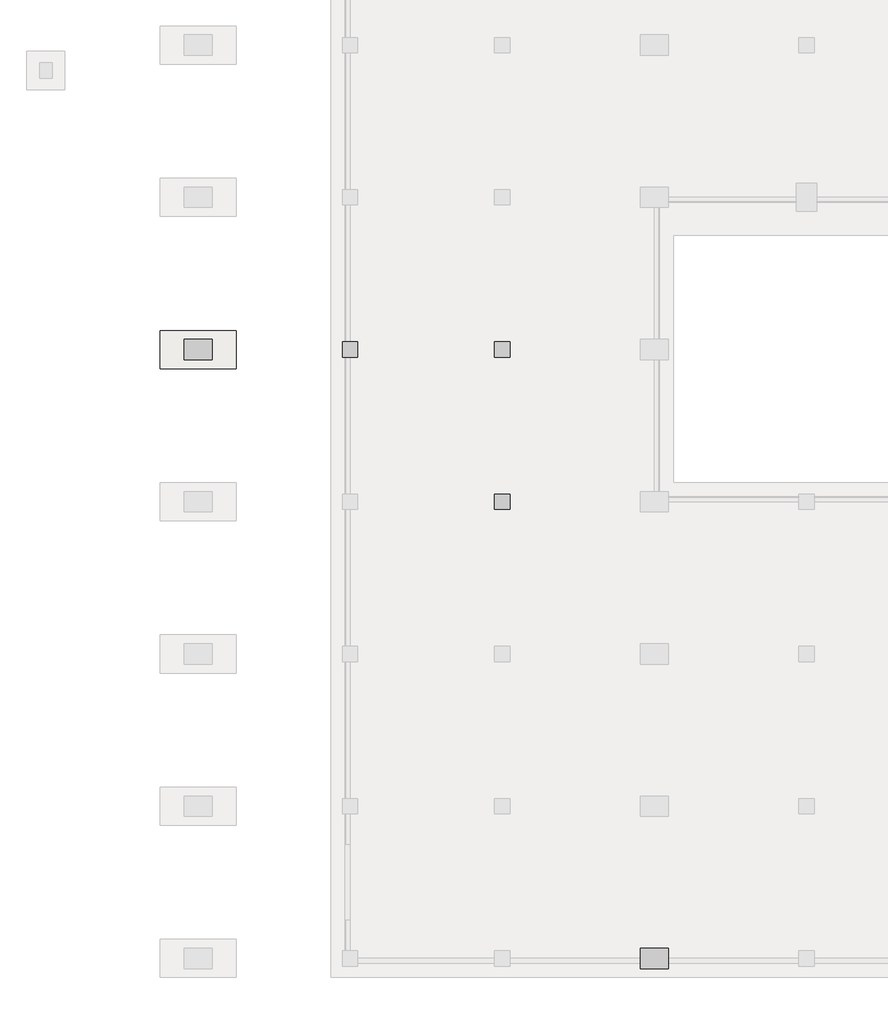
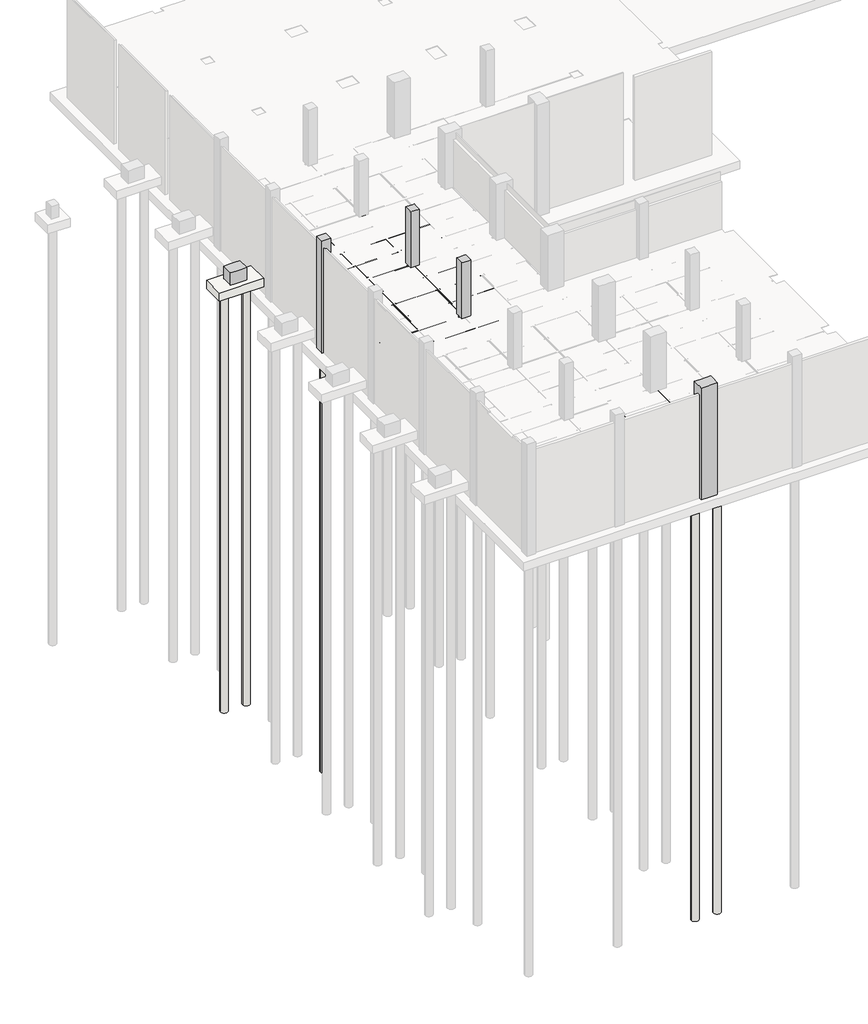
# Not in any storey, part 3 of 16: 28 beams, 6 slabs, 5 columns.
"""IFC4 building model written with IfcOpenShell, lengths in millimetres."""

from ifc_helpers import new_model, si_unit, point, frame, frame_2d, origin, place, context, project, spatial, polyline, circle_curve, trimmed, segment, composite_curve, outline, extrude, faceted_brep, element, save

model = new_model("IFC4")

# Units and contexts
model_context = context("Model", 3, world=origin())
ifc_project = project(units=[si_unit("LENGTHUNIT", "METRE", prefix="MILLI")], contexts=[model_context])

# Site, building
site = spatial("IfcSite", under=ifc_project)
building = spatial("IfcBuilding", under=site)

# Beams
placement = place(None, origin())
element("IfcBeam", 1, ObjectType="Steel Framing_C_KS : H_SB_AR_S02_C-150x75x6.5x10_J1", at=placement, inside=building, context=model_context, shape_type="SweptSolid", body=[
    extrude(outline(composite_curve([segment(polyline([(-43477.2, -3800.0381366), (-43477.2, -3950.0381366), (-43552.2, -3950.0381366)]), True, "CONTINUOUS"), segment(trimmed(circle_curve(frame_2d((-43542.2, -3950.0381366)), 10.0), [point((-43552.2, -3950.0381366))], [point((-43542.2, -3940.0381366))], False, "CARTESIAN"), True, "CONTINUOUS"), segment(polyline([(-43542.2, -3940.0381366), (-43483.7, -3930.7726469), (-43483.7, -3819.3036264), (-43542.2, -3810.0381366)]), True, "CONTINUOUS"), segment(trimmed(circle_curve(frame_2d((-43542.2, -3800.0381366)), 10.0), [point((-43542.2, -3810.0381366))], [point((-43552.2, -3800.0381366))], False, "CARTESIAN"), True, "CONTINUOUS"), segment(polyline([(-43552.2, -3800.0381366), (-43477.2, -3800.0381366)]), True, "CONTINUOUS")], self_intersect=False)), frame((27112.7, 0.0, 0.0), z_axis=(1.0, 0.0, 0.0), x_axis=(0.0, 1.0, 0.0)), (0.0, 0.0, 1.0), 2774.6),
])
element("IfcBeam", 2, ObjectType="Steel Framing_C_KS : H_SB_AR_S02_C-150x75x6.5x10_J1", at=placement, inside=building, context=model_context, shape_type="SweptSolid", body=[
    extrude(outline(composite_curve([segment(polyline([(-43477.2, -3800.0381366), (-43477.2, -3950.0381366), (-43552.2, -3950.0381366)]), True, "CONTINUOUS"), segment(trimmed(circle_curve(frame_2d((-43542.2, -3950.0381366)), 10.0), [point((-43552.2, -3950.0381366))], [point((-43542.2, -3940.0381366))], False, "CARTESIAN"), True, "CONTINUOUS"), segment(polyline([(-43542.2, -3940.0381366), (-43483.7, -3930.7726469), (-43483.7, -3819.3036264), (-43542.2, -3810.0381366)]), True, "CONTINUOUS"), segment(trimmed(circle_curve(frame_2d((-43542.2, -3800.0381366)), 10.0), [point((-43542.2, -3810.0381366))], [point((-43552.2, -3800.0381366))], False, "CARTESIAN"), True, "CONTINUOUS"), segment(polyline([(-43552.2, -3800.0381366), (-43477.2, -3800.0381366)]), True, "CONTINUOUS")], self_intersect=False)), frame((30112.7, 0.0, 0.0), z_axis=(1.0, 0.0, 0.0), x_axis=(0.0, 1.0, 0.0)), (0.0, 0.0, 1.0), 2774.6),
])
element("IfcBeam", 3, ObjectType="Steel Framing_H_KS : H_SB_AR_S02_H-400x200x8x13_BSG2", at=placement, inside=building, context=model_context, shape_type="SweptSolid", body=[
    extrude(outline(composite_curve([segment(polyline([(-4187.0381366, 35900.0), (-4200.0381366, 35900.0), (-4200.0381366, 36100.0), (-4187.0381366, 36100.0), (-4187.0381366, 36020.0)]), True, "CONTINUOUS"), segment(trimmed(circle_curve(frame_2d((-4171.0381366, 36020.0)), 16.0), [point((-4187.0381366, 36020.0))], [point((-4171.0381366, 36004.0))], True, "CARTESIAN"), True, "CONTINUOUS"), segment(polyline([(-4171.0381366, 36004.0), (-3829.0381366, 36004.0)]), True, "CONTINUOUS"), segment(trimmed(circle_curve(frame_2d((-3829.0381366, 36020.0)), 16.0), [point((-3829.0381366, 36004.0))], [point((-3813.0381366, 36020.0))], True, "CARTESIAN"), True, "CONTINUOUS"), segment(polyline([(-3813.0381366, 36020.0), (-3813.0381366, 36100.0), (-3800.0381366, 36100.0), (-3800.0381366, 35900.0), (-3813.0381366, 35900.0), (-3813.0381366, 35980.0)]), True, "CONTINUOUS"), segment(trimmed(circle_curve(frame_2d((-3829.0381366, 35980.0)), 16.0), [point((-3813.0381366, 35980.0))], [point((-3829.0381366, 35996.0))], True, "CARTESIAN"), True, "CONTINUOUS"), segment(polyline([(-3829.0381366, 35996.0), (-4171.0381366, 35996.0)]), True, "CONTINUOUS"), segment(trimmed(circle_curve(frame_2d((-4171.0381366, 35980.0)), 16.0), [point((-4171.0381366, 35996.0))], [point((-4187.0381366, 35980.0))], True, "CARTESIAN"), True, "CONTINUOUS"), segment(polyline([(-4187.0381366, 35980.0), (-4187.0381366, 35900.0)]), True, "CONTINUOUS")], self_intersect=False)), frame((0.0, -59587.3, 0.0), z_axis=(0.0, 1.0, 0.0), x_axis=(0.0, 0.0, 1.0)), (0.0, 0.0, 1.0), 5174.6),
])
element("IfcBeam", 4, ObjectType="Steel Framing_H_KS : H_SB_AR_S02_H-400x200x8x13_BSB1", at=placement, inside=building, context=model_context, shape_type="SweptSolid", body=[
    extrude(outline(composite_curve([segment(polyline([(-4187.0381366, 32900.0), (-4200.0381366, 32900.0), (-4200.0381366, 33100.0), (-4187.0381366, 33100.0), (-4187.0381366, 33020.0)]), True, "CONTINUOUS"), segment(trimmed(circle_curve(frame_2d((-4171.0381366, 33020.0)), 16.0), [point((-4187.0381366, 33020.0))], [point((-4171.0381366, 33004.0))], True, "CARTESIAN"), True, "CONTINUOUS"), segment(polyline([(-4171.0381366, 33004.0), (-3829.0381366, 33004.0)]), True, "CONTINUOUS"), segment(trimmed(circle_curve(frame_2d((-3829.0381366, 33020.0)), 16.0), [point((-3829.0381366, 33004.0))], [point((-3813.0381366, 33020.0))], True, "CARTESIAN"), True, "CONTINUOUS"), segment(polyline([(-3813.0381366, 33020.0), (-3813.0381366, 33100.0), (-3800.0381366, 33100.0), (-3800.0381366, 32900.0), (-3813.0381366, 32900.0), (-3813.0381366, 32980.0)]), True, "CONTINUOUS"), segment(trimmed(circle_curve(frame_2d((-3829.0381366, 32980.0)), 16.0), [point((-3813.0381366, 32980.0))], [point((-3829.0381366, 32996.0))], True, "CARTESIAN"), True, "CONTINUOUS"), segment(polyline([(-3829.0381366, 32996.0), (-4171.0381366, 32996.0)]), True, "CONTINUOUS"), segment(trimmed(circle_curve(frame_2d((-4171.0381366, 32980.0)), 16.0), [point((-4171.0381366, 32996.0))], [point((-4187.0381366, 32980.0))], True, "CARTESIAN"), True, "CONTINUOUS"), segment(polyline([(-4187.0381366, 32980.0), (-4187.0381366, 32900.0)]), True, "CONTINUOUS")], self_intersect=False)), frame((0.0, -60000.0, 0.0), z_axis=(0.0, 1.0, 0.0), x_axis=(0.0, 0.0, 1.0)), (0.0, 0.0, 1.0), 5887.3),
])
element("IfcBeam", 5, ObjectType="Steel Framing_C_KS : H_SB_AR_S02_C-150x75x6.5x10_J1", at=placement, inside=building, context=model_context, shape_type="SweptSolid", body=[
    extrude(outline(composite_curve([segment(polyline([(-56977.2, -3800.0381366), (-56977.2, -3950.0381366), (-57052.2, -3950.0381366)]), True, "CONTINUOUS"), segment(trimmed(circle_curve(frame_2d((-57042.2, -3950.0381366)), 10.0), [point((-57052.2, -3950.0381366))], [point((-57042.2, -3940.0381366))], False, "CARTESIAN"), True, "CONTINUOUS"), segment(polyline([(-57042.2, -3940.0381366), (-56983.7, -3930.7726469), (-56983.7, -3819.3036264), (-57042.2, -3810.0381366)]), True, "CONTINUOUS"), segment(trimmed(circle_curve(frame_2d((-57042.2, -3800.0381366)), 10.0), [point((-57042.2, -3810.0381366))], [point((-57052.2, -3800.0381366))], False, "CARTESIAN"), True, "CONTINUOUS"), segment(polyline([(-57052.2, -3800.0381366), (-56977.2, -3800.0381366)]), True, "CONTINUOUS")], self_intersect=False)), frame((33112.7, 0.0, 0.0), z_axis=(1.0, 0.0, 0.0), x_axis=(0.0, 1.0, 0.0)), (0.0, 0.0, 1.0), 2774.6),
])
element("IfcBeam", 6, ObjectType="Steel Framing_C_KS : H_SB_AR_S02_C-150x75x6.5x10_J1", at=placement, inside=building, context=model_context, shape_type="SweptSolid", body=[
    extrude(outline(composite_curve([segment(polyline([(-58477.2, -3800.0381366), (-58477.2, -3950.0381366), (-58552.2, -3950.0381366)]), True, "CONTINUOUS"), segment(trimmed(circle_curve(frame_2d((-58542.2, -3950.0381366)), 10.0), [point((-58552.2, -3950.0381366))], [point((-58542.2, -3940.0381366))], False, "CARTESIAN"), True, "CONTINUOUS"), segment(polyline([(-58542.2, -3940.0381366), (-58483.7, -3930.7726469), (-58483.7, -3819.3036264), (-58542.2, -3810.0381366)]), True, "CONTINUOUS"), segment(trimmed(circle_curve(frame_2d((-58542.2, -3800.0381366)), 10.0), [point((-58542.2, -3810.0381366))], [point((-58552.2, -3800.0381366))], False, "CARTESIAN"), True, "CONTINUOUS"), segment(polyline([(-58552.2, -3800.0381366), (-58477.2, -3800.0381366)]), True, "CONTINUOUS")], self_intersect=False)), frame((33112.7, 0.0, 0.0), z_axis=(1.0, 0.0, 0.0), x_axis=(0.0, 1.0, 0.0)), (0.0, 0.0, 1.0), 2774.6),
])
element("IfcBeam", 7, ObjectType="Steel Framing_C_KS : H_SB_AR_S02_C-150x75x6.5x10_J1", at=placement, inside=building, context=model_context, shape_type="SweptSolid", body=[
    extrude(outline(composite_curve([segment(polyline([(-56977.2, -3800.0381366), (-56977.2, -3950.0381366), (-57052.2, -3950.0381366)]), True, "CONTINUOUS"), segment(trimmed(circle_curve(frame_2d((-57042.2, -3950.0381366)), 10.0), [point((-57052.2, -3950.0381366))], [point((-57042.2, -3940.0381366))], False, "CARTESIAN"), True, "CONTINUOUS"), segment(polyline([(-57042.2, -3940.0381366), (-56983.7, -3930.7726469), (-56983.7, -3819.3036264), (-57042.2, -3810.0381366)]), True, "CONTINUOUS"), segment(trimmed(circle_curve(frame_2d((-57042.2, -3800.0381366)), 10.0), [point((-57042.2, -3810.0381366))], [point((-57052.2, -3800.0381366))], False, "CARTESIAN"), True, "CONTINUOUS"), segment(polyline([(-57052.2, -3800.0381366), (-56977.2, -3800.0381366)]), True, "CONTINUOUS")], self_intersect=False)), frame((36112.7, 0.0, 0.0), z_axis=(1.0, 0.0, 0.0), x_axis=(0.0, 1.0, 0.0)), (0.0, 0.0, 1.0), 2774.6),
])
element("IfcBeam", 8, ObjectType="Steel Framing_C_KS : H_SB_AR_S02_C-150x75x6.5x10_J1", at=placement, inside=building, context=model_context, shape_type="SweptSolid", body=[
    extrude(outline(composite_curve([segment(polyline([(-58477.2, -3800.0381366), (-58477.2, -3950.0381366), (-58552.2, -3950.0381366)]), True, "CONTINUOUS"), segment(trimmed(circle_curve(frame_2d((-58542.2, -3950.0381366)), 10.0), [point((-58552.2, -3950.0381366))], [point((-58542.2, -3940.0381366))], False, "CARTESIAN"), True, "CONTINUOUS"), segment(polyline([(-58542.2, -3940.0381366), (-58483.7, -3930.7726469), (-58483.7, -3819.3036264), (-58542.2, -3810.0381366)]), True, "CONTINUOUS"), segment(trimmed(circle_curve(frame_2d((-58542.2, -3800.0381366)), 10.0), [point((-58542.2, -3810.0381366))], [point((-58552.2, -3800.0381366))], False, "CARTESIAN"), True, "CONTINUOUS"), segment(polyline([(-58552.2, -3800.0381366), (-58477.2, -3800.0381366)]), True, "CONTINUOUS")], self_intersect=False)), frame((36112.7, 0.0, 0.0), z_axis=(1.0, 0.0, 0.0), x_axis=(0.0, 1.0, 0.0)), (0.0, 0.0, 1.0), 2774.6),
])
element("IfcBeam", 9, ObjectType="Steel Framing_H_KS : H_SB_AR_S02_H-400x200x8x13_BSG1", at=placement, inside=building, context=model_context, shape_type="SweptSolid", body=[
    extrude(outline(composite_curve([segment(polyline([(-35900.0, -4187.0381366), (-35900.0, -4200.0381366), (-36100.0, -4200.0381366), (-36100.0, -4187.0381366), (-36020.0, -4187.0381366)]), True, "CONTINUOUS"), segment(trimmed(circle_curve(frame_2d((-36020.0, -4171.0381366)), 16.0), [point((-36020.0, -4187.0381366))], [point((-36004.0, -4171.0381366))], True, "CARTESIAN"), True, "CONTINUOUS"), segment(polyline([(-36004.0, -4171.0381366), (-36004.0, -3829.0381366)]), True, "CONTINUOUS"), segment(trimmed(circle_curve(frame_2d((-36020.0, -3829.0381366)), 16.0), [point((-36004.0, -3829.0381366))], [point((-36020.0, -3813.0381366))], True, "CARTESIAN"), True, "CONTINUOUS"), segment(polyline([(-36020.0, -3813.0381366), (-36100.0, -3813.0381366), (-36100.0, -3800.0381366), (-35900.0, -3800.0381366), (-35900.0, -3813.0381366), (-35980.0, -3813.0381366)]), True, "CONTINUOUS"), segment(trimmed(circle_curve(frame_2d((-35980.0, -3829.0381366)), 16.0), [point((-35980.0, -3813.0381366))], [point((-35996.0, -3829.0381366))], True, "CARTESIAN"), True, "CONTINUOUS"), segment(polyline([(-35996.0, -3829.0381366), (-35996.0, -4171.0381366)]), True, "CONTINUOUS"), segment(trimmed(circle_curve(frame_2d((-35980.0, -4171.0381366)), 16.0), [point((-35996.0, -4171.0381366))], [point((-35980.0, -4187.0381366))], True, "CARTESIAN"), True, "CONTINUOUS"), segment(polyline([(-35980.0, -4187.0381366), (-35900.0, -4187.0381366)]), True, "CONTINUOUS")], self_intersect=False)), frame((24312.7, 0.0, 0.0), z_axis=(1.0, 0.0, 0.0), x_axis=(0.0, 1.0, 0.0)), (0.0, 0.0, 1.0), 5374.6),
])
element("IfcBeam", 10, ObjectType="Steel Framing_H_KS : H_SB_AR_S02_H-400x200x8x13_BSG2", at=placement, inside=building, context=model_context, shape_type="SweptSolid", body=[
    extrude(outline(composite_curve([segment(polyline([(-4187.0381366, 29900.0), (-4200.0381366, 29900.0), (-4200.0381366, 30100.0), (-4187.0381366, 30100.0), (-4187.0381366, 30020.0)]), True, "CONTINUOUS"), segment(trimmed(circle_curve(frame_2d((-4171.0381366, 30020.0)), 16.0), [point((-4187.0381366, 30020.0))], [point((-4171.0381366, 30004.0))], True, "CARTESIAN"), True, "CONTINUOUS"), segment(polyline([(-4171.0381366, 30004.0), (-3829.0381366, 30004.0)]), True, "CONTINUOUS"), segment(trimmed(circle_curve(frame_2d((-3829.0381366, 30020.0)), 16.0), [point((-3829.0381366, 30004.0))], [point((-3813.0381366, 30020.0))], True, "CARTESIAN"), True, "CONTINUOUS"), segment(polyline([(-3813.0381366, 30020.0), (-3813.0381366, 30100.0), (-3800.0381366, 30100.0), (-3800.0381366, 29900.0), (-3813.0381366, 29900.0), (-3813.0381366, 29980.0)]), True, "CONTINUOUS"), segment(trimmed(circle_curve(frame_2d((-3829.0381366, 29980.0)), 16.0), [point((-3813.0381366, 29980.0))], [point((-3829.0381366, 29996.0))], True, "CARTESIAN"), True, "CONTINUOUS"), segment(polyline([(-3829.0381366, 29996.0), (-4171.0381366, 29996.0)]), True, "CONTINUOUS"), segment(trimmed(circle_curve(frame_2d((-4171.0381366, 29980.0)), 16.0), [point((-4171.0381366, 29996.0))], [point((-4187.0381366, 29980.0))], True, "CARTESIAN"), True, "CONTINUOUS"), segment(polyline([(-4187.0381366, 29980.0), (-4187.0381366, 29900.0)]), True, "CONTINUOUS")], self_intersect=False)), frame((0.0, -35687.3, 0.0), z_axis=(0.0, 1.0, 0.0), x_axis=(0.0, 0.0, 1.0)), (0.0, 0.0, 1.0), 5374.6),
])
element("IfcBeam", 11, ObjectType="Steel Framing_H_KS : H_SB_AR_S02_H-400x200x8x13_BSB1", at=placement, inside=building, context=model_context, shape_type="SweptSolid", body=[
    extrude(outline(composite_curve([segment(polyline([(-4187.0381366, 26900.0), (-4200.0381366, 26900.0), (-4200.0381366, 27100.0), (-4187.0381366, 27100.0), (-4187.0381366, 27020.0)]), True, "CONTINUOUS"), segment(trimmed(circle_curve(frame_2d((-4171.0381366, 27020.0)), 16.0), [point((-4187.0381366, 27020.0))], [point((-4171.0381366, 27004.0))], True, "CARTESIAN"), True, "CONTINUOUS"), segment(polyline([(-4171.0381366, 27004.0), (-3829.0381366, 27004.0)]), True, "CONTINUOUS"), segment(trimmed(circle_curve(frame_2d((-3829.0381366, 27020.0)), 16.0), [point((-3829.0381366, 27004.0))], [point((-3813.0381366, 27020.0))], True, "CARTESIAN"), True, "CONTINUOUS"), segment(polyline([(-3813.0381366, 27020.0), (-3813.0381366, 27100.0), (-3800.0381366, 27100.0), (-3800.0381366, 26900.0), (-3813.0381366, 26900.0), (-3813.0381366, 26980.0)]), True, "CONTINUOUS"), segment(trimmed(circle_curve(frame_2d((-3829.0381366, 26980.0)), 16.0), [point((-3813.0381366, 26980.0))], [point((-3829.0381366, 26996.0))], True, "CARTESIAN"), True, "CONTINUOUS"), segment(polyline([(-3829.0381366, 26996.0), (-4171.0381366, 26996.0)]), True, "CONTINUOUS"), segment(trimmed(circle_curve(frame_2d((-4171.0381366, 26980.0)), 16.0), [point((-4171.0381366, 26996.0))], [point((-4187.0381366, 26980.0))], True, "CARTESIAN"), True, "CONTINUOUS"), segment(polyline([(-4187.0381366, 26980.0), (-4187.0381366, 26900.0)]), True, "CONTINUOUS")], self_intersect=False)), frame((0.0, -35887.3, 0.0), z_axis=(0.0, 1.0, 0.0), x_axis=(0.0, 0.0, 1.0)), (0.0, 0.0, 1.0), 5774.6),
])
element("IfcBeam", 12, ObjectType="Steel Framing_C_KS : H_SB_AR_S02_C-150x75x6.5x10_J1", at=placement, inside=building, context=model_context, shape_type="SweptSolid", body=[
    extrude(outline(composite_curve([segment(polyline([(-32977.2, -3800.0381366), (-32977.2, -3950.0381366), (-33052.2, -3950.0381366)]), True, "CONTINUOUS"), segment(trimmed(circle_curve(frame_2d((-33042.2, -3950.0381366)), 10.0), [point((-33052.2, -3950.0381366))], [point((-33042.2, -3940.0381366))], False, "CARTESIAN"), True, "CONTINUOUS"), segment(polyline([(-33042.2, -3940.0381366), (-32983.7, -3930.7726469), (-32983.7, -3819.3036264), (-33042.2, -3810.0381366)]), True, "CONTINUOUS"), segment(trimmed(circle_curve(frame_2d((-33042.2, -3800.0381366)), 10.0), [point((-33042.2, -3810.0381366))], [point((-33052.2, -3800.0381366))], False, "CARTESIAN"), True, "CONTINUOUS"), segment(polyline([(-33052.2, -3800.0381366), (-32977.2, -3800.0381366)]), True, "CONTINUOUS")], self_intersect=False)), frame((24000.0, 0.0, 0.0), z_axis=(1.0, 0.0, 0.0), x_axis=(0.0, 1.0, 0.0)), (0.0, 0.0, 1.0), 2887.3),
])
element("IfcBeam", 13, ObjectType="Steel Framing_C_KS : H_SB_AR_S02_C-150x75x6.5x10_J1", at=placement, inside=building, context=model_context, shape_type="SweptSolid", body=[
    extrude(outline(composite_curve([segment(polyline([(-34477.2, -3800.0381366), (-34477.2, -3950.0381366), (-34552.2, -3950.0381366)]), True, "CONTINUOUS"), segment(trimmed(circle_curve(frame_2d((-34542.2, -3950.0381366)), 10.0), [point((-34552.2, -3950.0381366))], [point((-34542.2, -3940.0381366))], False, "CARTESIAN"), True, "CONTINUOUS"), segment(polyline([(-34542.2, -3940.0381366), (-34483.7, -3930.7726469), (-34483.7, -3819.3036264), (-34542.2, -3810.0381366)]), True, "CONTINUOUS"), segment(trimmed(circle_curve(frame_2d((-34542.2, -3800.0381366)), 10.0), [point((-34542.2, -3810.0381366))], [point((-34552.2, -3800.0381366))], False, "CARTESIAN"), True, "CONTINUOUS"), segment(polyline([(-34552.2, -3800.0381366), (-34477.2, -3800.0381366)]), True, "CONTINUOUS")], self_intersect=False)), frame((24000.0, 0.0, 0.0), z_axis=(1.0, 0.0, 0.0), x_axis=(0.0, 1.0, 0.0)), (0.0, 0.0, 1.0), 2887.3),
])
element("IfcBeam", 14, ObjectType="Steel Framing_C_KS : H_SB_AR_S02_C-150x75x6.5x10_J1", at=placement, inside=building, context=model_context, shape_type="SweptSolid", body=[
    extrude(outline(composite_curve([segment(polyline([(-32977.2, -3800.0381366), (-32977.2, -3950.0381366), (-33052.2, -3950.0381366)]), True, "CONTINUOUS"), segment(trimmed(circle_curve(frame_2d((-33042.2, -3950.0381366)), 10.0), [point((-33052.2, -3950.0381366))], [point((-33042.2, -3940.0381366))], False, "CARTESIAN"), True, "CONTINUOUS"), segment(polyline([(-33042.2, -3940.0381366), (-32983.7, -3930.7726469), (-32983.7, -3819.3036264), (-33042.2, -3810.0381366)]), True, "CONTINUOUS"), segment(trimmed(circle_curve(frame_2d((-33042.2, -3800.0381366)), 10.0), [point((-33042.2, -3810.0381366))], [point((-33052.2, -3800.0381366))], False, "CARTESIAN"), True, "CONTINUOUS"), segment(polyline([(-33052.2, -3800.0381366), (-32977.2, -3800.0381366)]), True, "CONTINUOUS")], self_intersect=False)), frame((27112.7, 0.0, 0.0), z_axis=(1.0, 0.0, 0.0), x_axis=(0.0, 1.0, 0.0)), (0.0, 0.0, 1.0), 2774.6),
])
element("IfcBeam", 15, ObjectType="Steel Framing_C_KS : H_SB_AR_S02_C-150x75x6.5x10_J1", at=placement, inside=building, context=model_context, shape_type="SweptSolid", body=[
    extrude(outline(composite_curve([segment(polyline([(-34477.2, -3800.0381366), (-34477.2, -3950.0381366), (-34552.2, -3950.0381366)]), True, "CONTINUOUS"), segment(trimmed(circle_curve(frame_2d((-34542.2, -3950.0381366)), 10.0), [point((-34552.2, -3950.0381366))], [point((-34542.2, -3940.0381366))], False, "CARTESIAN"), True, "CONTINUOUS"), segment(polyline([(-34542.2, -3940.0381366), (-34483.7, -3930.7726469), (-34483.7, -3819.3036264), (-34542.2, -3810.0381366)]), True, "CONTINUOUS"), segment(trimmed(circle_curve(frame_2d((-34542.2, -3800.0381366)), 10.0), [point((-34542.2, -3810.0381366))], [point((-34552.2, -3800.0381366))], False, "CARTESIAN"), True, "CONTINUOUS"), segment(polyline([(-34552.2, -3800.0381366), (-34477.2, -3800.0381366)]), True, "CONTINUOUS")], self_intersect=False)), frame((27112.7, 0.0, 0.0), z_axis=(1.0, 0.0, 0.0), x_axis=(0.0, 1.0, 0.0)), (0.0, 0.0, 1.0), 2774.6),
])
element("IfcBeam", 16, ObjectType="Steel Framing_C_KS : H_SB_AR_S02_C-150x75x6.5x10_J1", at=placement, inside=building, context=model_context, shape_type="SweptSolid", body=[
    extrude(outline(composite_curve([segment(polyline([(-32977.2, -3800.0381366), (-32977.2, -3950.0381366), (-33052.2, -3950.0381366)]), True, "CONTINUOUS"), segment(trimmed(circle_curve(frame_2d((-33042.2, -3950.0381366)), 10.0), [point((-33052.2, -3950.0381366))], [point((-33042.2, -3940.0381366))], False, "CARTESIAN"), True, "CONTINUOUS"), segment(polyline([(-33042.2, -3940.0381366), (-32983.7, -3930.7726469), (-32983.7, -3819.3036264), (-33042.2, -3810.0381366)]), True, "CONTINUOUS"), segment(trimmed(circle_curve(frame_2d((-33042.2, -3800.0381366)), 10.0), [point((-33042.2, -3810.0381366))], [point((-33052.2, -3800.0381366))], False, "CARTESIAN"), True, "CONTINUOUS"), segment(polyline([(-33052.2, -3800.0381366), (-32977.2, -3800.0381366)]), True, "CONTINUOUS")], self_intersect=False)), frame((30112.7, 0.0, 0.0), z_axis=(1.0, 0.0, 0.0), x_axis=(0.0, 1.0, 0.0)), (0.0, 0.0, 1.0), 2774.6),
])
element("IfcBeam", 17, ObjectType="Steel Framing_C_KS : H_SB_AR_S02_C-150x75x6.5x10_J1", at=placement, inside=building, context=model_context, shape_type="SweptSolid", body=[
    extrude(outline(composite_curve([segment(polyline([(-34477.2, -3800.0381366), (-34477.2, -3950.0381366), (-34552.2, -3950.0381366)]), True, "CONTINUOUS"), segment(trimmed(circle_curve(frame_2d((-34542.2, -3950.0381366)), 10.0), [point((-34552.2, -3950.0381366))], [point((-34542.2, -3940.0381366))], False, "CARTESIAN"), True, "CONTINUOUS"), segment(polyline([(-34542.2, -3940.0381366), (-34483.7, -3930.7726469), (-34483.7, -3819.3036264), (-34542.2, -3810.0381366)]), True, "CONTINUOUS"), segment(trimmed(circle_curve(frame_2d((-34542.2, -3800.0381366)), 10.0), [point((-34542.2, -3810.0381366))], [point((-34552.2, -3800.0381366))], False, "CARTESIAN"), True, "CONTINUOUS"), segment(polyline([(-34552.2, -3800.0381366), (-34477.2, -3800.0381366)]), True, "CONTINUOUS")], self_intersect=False)), frame((30112.7, 0.0, 0.0), z_axis=(1.0, 0.0, 0.0), x_axis=(0.0, 1.0, 0.0)), (0.0, 0.0, 1.0), 2774.6),
])
element("IfcBeam", 18, ObjectType="Steel Framing_H_KS : H_SB_AR_S02_H-400x200x8x13_BSG1", at=placement, inside=building, context=model_context, shape_type="SweptSolid", body=[
    extrude(outline(composite_curve([segment(polyline([(-41900.0, -4187.0381366), (-41900.0, -4200.0381366), (-42100.0, -4200.0381366), (-42100.0, -4187.0381366), (-42020.0, -4187.0381366)]), True, "CONTINUOUS"), segment(trimmed(circle_curve(frame_2d((-42020.0, -4171.0381366)), 16.0), [point((-42020.0, -4187.0381366))], [point((-42004.0, -4171.0381366))], True, "CARTESIAN"), True, "CONTINUOUS"), segment(polyline([(-42004.0, -4171.0381366), (-42004.0, -3829.0381366)]), True, "CONTINUOUS"), segment(trimmed(circle_curve(frame_2d((-42020.0, -3829.0381366)), 16.0), [point((-42004.0, -3829.0381366))], [point((-42020.0, -3813.0381366))], True, "CARTESIAN"), True, "CONTINUOUS"), segment(polyline([(-42020.0, -3813.0381366), (-42100.0, -3813.0381366), (-42100.0, -3800.0381366), (-41900.0, -3800.0381366), (-41900.0, -3813.0381366), (-41980.0, -3813.0381366)]), True, "CONTINUOUS"), segment(trimmed(circle_curve(frame_2d((-41980.0, -3829.0381366)), 16.0), [point((-41980.0, -3813.0381366))], [point((-41996.0, -3829.0381366))], True, "CARTESIAN"), True, "CONTINUOUS"), segment(polyline([(-41996.0, -3829.0381366), (-41996.0, -4171.0381366)]), True, "CONTINUOUS"), segment(trimmed(circle_curve(frame_2d((-41980.0, -4171.0381366)), 16.0), [point((-41996.0, -4171.0381366))], [point((-41980.0, -4187.0381366))], True, "CARTESIAN"), True, "CONTINUOUS"), segment(polyline([(-41980.0, -4187.0381366), (-41900.0, -4187.0381366)]), True, "CONTINUOUS")], self_intersect=False)), frame((24312.7, 0.0, 0.0), z_axis=(1.0, 0.0, 0.0), x_axis=(0.0, 1.0, 0.0)), (0.0, 0.0, 1.0), 5374.6),
])
element("IfcBeam", 19, ObjectType="Steel Framing_H_KS : H_SB_AR_S02_H-400x200x8x13_BSG2", at=placement, inside=building, context=model_context, shape_type="SweptSolid", body=[
    extrude(outline(composite_curve([segment(polyline([(-4187.0381366, 29900.0), (-4200.0381366, 29900.0), (-4200.0381366, 30100.0), (-4187.0381366, 30100.0), (-4187.0381366, 30020.0)]), True, "CONTINUOUS"), segment(trimmed(circle_curve(frame_2d((-4171.0381366, 30020.0)), 16.0), [point((-4187.0381366, 30020.0))], [point((-4171.0381366, 30004.0))], True, "CARTESIAN"), True, "CONTINUOUS"), segment(polyline([(-4171.0381366, 30004.0), (-3829.0381366, 30004.0)]), True, "CONTINUOUS"), segment(trimmed(circle_curve(frame_2d((-3829.0381366, 30020.0)), 16.0), [point((-3829.0381366, 30004.0))], [point((-3813.0381366, 30020.0))], True, "CARTESIAN"), True, "CONTINUOUS"), segment(polyline([(-3813.0381366, 30020.0), (-3813.0381366, 30100.0), (-3800.0381366, 30100.0), (-3800.0381366, 29900.0), (-3813.0381366, 29900.0), (-3813.0381366, 29980.0)]), True, "CONTINUOUS"), segment(trimmed(circle_curve(frame_2d((-3829.0381366, 29980.0)), 16.0), [point((-3813.0381366, 29980.0))], [point((-3829.0381366, 29996.0))], True, "CARTESIAN"), True, "CONTINUOUS"), segment(polyline([(-3829.0381366, 29996.0), (-4171.0381366, 29996.0)]), True, "CONTINUOUS"), segment(trimmed(circle_curve(frame_2d((-4171.0381366, 29980.0)), 16.0), [point((-4171.0381366, 29996.0))], [point((-4187.0381366, 29980.0))], True, "CARTESIAN"), True, "CONTINUOUS"), segment(polyline([(-4187.0381366, 29980.0), (-4187.0381366, 29900.0)]), True, "CONTINUOUS")], self_intersect=False)), frame((0.0, -41687.3, 0.0), z_axis=(0.0, 1.0, 0.0), x_axis=(0.0, 0.0, 1.0)), (0.0, 0.0, 1.0), 5374.6),
])
element("IfcBeam", 20, ObjectType="Steel Framing_H_KS : H_SB_AR_S02_H-400x200x8x13_BSB1", at=placement, inside=building, context=model_context, shape_type="SweptSolid", body=[
    extrude(outline(composite_curve([segment(polyline([(-4187.0381366, 26900.0), (-4200.0381366, 26900.0), (-4200.0381366, 27100.0), (-4187.0381366, 27100.0), (-4187.0381366, 27020.0)]), True, "CONTINUOUS"), segment(trimmed(circle_curve(frame_2d((-4171.0381366, 27020.0)), 16.0), [point((-4187.0381366, 27020.0))], [point((-4171.0381366, 27004.0))], True, "CARTESIAN"), True, "CONTINUOUS"), segment(polyline([(-4171.0381366, 27004.0), (-3829.0381366, 27004.0)]), True, "CONTINUOUS"), segment(trimmed(circle_curve(frame_2d((-3829.0381366, 27020.0)), 16.0), [point((-3829.0381366, 27004.0))], [point((-3813.0381366, 27020.0))], True, "CARTESIAN"), True, "CONTINUOUS"), segment(polyline([(-3813.0381366, 27020.0), (-3813.0381366, 27100.0), (-3800.0381366, 27100.0), (-3800.0381366, 26900.0), (-3813.0381366, 26900.0), (-3813.0381366, 26980.0)]), True, "CONTINUOUS"), segment(trimmed(circle_curve(frame_2d((-3829.0381366, 26980.0)), 16.0), [point((-3813.0381366, 26980.0))], [point((-3829.0381366, 26996.0))], True, "CARTESIAN"), True, "CONTINUOUS"), segment(polyline([(-3829.0381366, 26996.0), (-4171.0381366, 26996.0)]), True, "CONTINUOUS"), segment(trimmed(circle_curve(frame_2d((-4171.0381366, 26980.0)), 16.0), [point((-4171.0381366, 26996.0))], [point((-4187.0381366, 26980.0))], True, "CARTESIAN"), True, "CONTINUOUS"), segment(polyline([(-4187.0381366, 26980.0), (-4187.0381366, 26900.0)]), True, "CONTINUOUS")], self_intersect=False)), frame((0.0, -41887.3, 0.0), z_axis=(0.0, 1.0, 0.0), x_axis=(0.0, 0.0, 1.0)), (0.0, 0.0, 1.0), 5774.6),
])
element("IfcBeam", 21, ObjectType="Steel Framing_C_KS : H_SB_AR_S02_C-150x75x6.5x10_J1", at=placement, inside=building, context=model_context, shape_type="SweptSolid", body=[
    extrude(outline(composite_curve([segment(polyline([(-38977.2, -3800.0381366), (-38977.2, -3950.0381366), (-39052.2, -3950.0381366)]), True, "CONTINUOUS"), segment(trimmed(circle_curve(frame_2d((-39042.2, -3950.0381366)), 10.0), [point((-39052.2, -3950.0381366))], [point((-39042.2, -3940.0381366))], False, "CARTESIAN"), True, "CONTINUOUS"), segment(polyline([(-39042.2, -3940.0381366), (-38983.7, -3930.7726469), (-38983.7, -3819.3036264), (-39042.2, -3810.0381366)]), True, "CONTINUOUS"), segment(trimmed(circle_curve(frame_2d((-39042.2, -3800.0381366)), 10.0), [point((-39042.2, -3810.0381366))], [point((-39052.2, -3800.0381366))], False, "CARTESIAN"), True, "CONTINUOUS"), segment(polyline([(-39052.2, -3800.0381366), (-38977.2, -3800.0381366)]), True, "CONTINUOUS")], self_intersect=False)), frame((24000.0, 0.0, 0.0), z_axis=(1.0, 0.0, 0.0), x_axis=(0.0, 1.0, 0.0)), (0.0, 0.0, 1.0), 2887.3),
])
element("IfcBeam", 22, ObjectType="Steel Framing_C_KS : H_SB_AR_S02_C-150x75x6.5x10_J1", at=placement, inside=building, context=model_context, shape_type="SweptSolid", body=[
    extrude(outline(composite_curve([segment(polyline([(-37477.2, -3800.0381366), (-37477.2, -3950.0381366), (-37552.2, -3950.0381366)]), True, "CONTINUOUS"), segment(trimmed(circle_curve(frame_2d((-37542.2, -3950.0381366)), 10.0), [point((-37552.2, -3950.0381366))], [point((-37542.2, -3940.0381366))], False, "CARTESIAN"), True, "CONTINUOUS"), segment(polyline([(-37542.2, -3940.0381366), (-37483.7, -3930.7726469), (-37483.7, -3819.3036264), (-37542.2, -3810.0381366)]), True, "CONTINUOUS"), segment(trimmed(circle_curve(frame_2d((-37542.2, -3800.0381366)), 10.0), [point((-37542.2, -3810.0381366))], [point((-37552.2, -3800.0381366))], False, "CARTESIAN"), True, "CONTINUOUS"), segment(polyline([(-37552.2, -3800.0381366), (-37477.2, -3800.0381366)]), True, "CONTINUOUS")], self_intersect=False)), frame((24000.0, 0.0, 0.0), z_axis=(1.0, 0.0, 0.0), x_axis=(0.0, 1.0, 0.0)), (0.0, 0.0, 1.0), 2887.3),
])
element("IfcBeam", 23, ObjectType="Steel Framing_C_KS : H_SB_AR_S02_C-150x75x6.5x10_J1", at=placement, inside=building, context=model_context, shape_type="SweptSolid", body=[
    extrude(outline(composite_curve([segment(polyline([(-38977.2, -3800.0381366), (-38977.2, -3950.0381366), (-39052.2, -3950.0381366)]), True, "CONTINUOUS"), segment(trimmed(circle_curve(frame_2d((-39042.2, -3950.0381366)), 10.0), [point((-39052.2, -3950.0381366))], [point((-39042.2, -3940.0381366))], False, "CARTESIAN"), True, "CONTINUOUS"), segment(polyline([(-39042.2, -3940.0381366), (-38983.7, -3930.7726469), (-38983.7, -3819.3036264), (-39042.2, -3810.0381366)]), True, "CONTINUOUS"), segment(trimmed(circle_curve(frame_2d((-39042.2, -3800.0381366)), 10.0), [point((-39042.2, -3810.0381366))], [point((-39052.2, -3800.0381366))], False, "CARTESIAN"), True, "CONTINUOUS"), segment(polyline([(-39052.2, -3800.0381366), (-38977.2, -3800.0381366)]), True, "CONTINUOUS")], self_intersect=False)), frame((27112.7, 0.0, 0.0), z_axis=(1.0, 0.0, 0.0), x_axis=(0.0, 1.0, 0.0)), (0.0, 0.0, 1.0), 2774.6),
])
element("IfcBeam", 24, ObjectType="Steel Framing_C_KS : H_SB_AR_S02_C-150x75x6.5x10_J1", at=placement, inside=building, context=model_context, shape_type="SweptSolid", body=[
    extrude(outline(composite_curve([segment(polyline([(-40477.2, -3800.0381366), (-40477.2, -3950.0381366), (-40552.2, -3950.0381366)]), True, "CONTINUOUS"), segment(trimmed(circle_curve(frame_2d((-40542.2, -3950.0381366)), 10.0), [point((-40552.2, -3950.0381366))], [point((-40542.2, -3940.0381366))], False, "CARTESIAN"), True, "CONTINUOUS"), segment(polyline([(-40542.2, -3940.0381366), (-40483.7, -3930.7726469), (-40483.7, -3819.3036264), (-40542.2, -3810.0381366)]), True, "CONTINUOUS"), segment(trimmed(circle_curve(frame_2d((-40542.2, -3800.0381366)), 10.0), [point((-40542.2, -3810.0381366))], [point((-40552.2, -3800.0381366))], False, "CARTESIAN"), True, "CONTINUOUS"), segment(polyline([(-40552.2, -3800.0381366), (-40477.2, -3800.0381366)]), True, "CONTINUOUS")], self_intersect=False)), frame((27112.7, 0.0, 0.0), z_axis=(1.0, 0.0, 0.0), x_axis=(0.0, 1.0, 0.0)), (0.0, 0.0, 1.0), 2774.6),
])
element("IfcBeam", 25, ObjectType="Steel Framing_C_KS : H_SB_AR_S02_C-150x75x6.5x10_J1", at=placement, inside=building, context=model_context, shape_type="SweptSolid", body=[
    extrude(outline(composite_curve([segment(polyline([(-37477.2, -3800.0381366), (-37477.2, -3950.0381366), (-37552.2, -3950.0381366)]), True, "CONTINUOUS"), segment(trimmed(circle_curve(frame_2d((-37542.2, -3950.0381366)), 10.0), [point((-37552.2, -3950.0381366))], [point((-37542.2, -3940.0381366))], False, "CARTESIAN"), True, "CONTINUOUS"), segment(polyline([(-37542.2, -3940.0381366), (-37483.7, -3930.7726469), (-37483.7, -3819.3036264), (-37542.2, -3810.0381366)]), True, "CONTINUOUS"), segment(trimmed(circle_curve(frame_2d((-37542.2, -3800.0381366)), 10.0), [point((-37542.2, -3810.0381366))], [point((-37552.2, -3800.0381366))], False, "CARTESIAN"), True, "CONTINUOUS"), segment(polyline([(-37552.2, -3800.0381366), (-37477.2, -3800.0381366)]), True, "CONTINUOUS")], self_intersect=False)), frame((27112.7, 0.0, 0.0), z_axis=(1.0, 0.0, 0.0), x_axis=(0.0, 1.0, 0.0)), (0.0, 0.0, 1.0), 2774.6),
])
element("IfcBeam", 26, ObjectType="Steel Framing_C_KS : H_SB_AR_S02_C-150x75x6.5x10_J1", at=placement, inside=building, context=model_context, shape_type="SweptSolid", body=[
    extrude(outline(composite_curve([segment(polyline([(-38977.2, -3800.0381366), (-38977.2, -3950.0381366), (-39052.2, -3950.0381366)]), True, "CONTINUOUS"), segment(trimmed(circle_curve(frame_2d((-39042.2, -3950.0381366)), 10.0), [point((-39052.2, -3950.0381366))], [point((-39042.2, -3940.0381366))], False, "CARTESIAN"), True, "CONTINUOUS"), segment(polyline([(-39042.2, -3940.0381366), (-38983.7, -3930.7726469), (-38983.7, -3819.3036264), (-39042.2, -3810.0381366)]), True, "CONTINUOUS"), segment(trimmed(circle_curve(frame_2d((-39042.2, -3800.0381366)), 10.0), [point((-39042.2, -3810.0381366))], [point((-39052.2, -3800.0381366))], False, "CARTESIAN"), True, "CONTINUOUS"), segment(polyline([(-39052.2, -3800.0381366), (-38977.2, -3800.0381366)]), True, "CONTINUOUS")], self_intersect=False)), frame((30112.7, 0.0, 0.0), z_axis=(1.0, 0.0, 0.0), x_axis=(0.0, 1.0, 0.0)), (0.0, 0.0, 1.0), 2774.6),
])
element("IfcBeam", 27, ObjectType="Steel Framing_C_KS : H_SB_AR_S02_C-150x75x6.5x10_J1", at=placement, inside=building, context=model_context, shape_type="SweptSolid", body=[
    extrude(outline(composite_curve([segment(polyline([(-40477.2, -3800.0381366), (-40477.2, -3950.0381366), (-40552.2, -3950.0381366)]), True, "CONTINUOUS"), segment(trimmed(circle_curve(frame_2d((-40542.2, -3950.0381366)), 10.0), [point((-40552.2, -3950.0381366))], [point((-40542.2, -3940.0381366))], False, "CARTESIAN"), True, "CONTINUOUS"), segment(polyline([(-40542.2, -3940.0381366), (-40483.7, -3930.7726469), (-40483.7, -3819.3036264), (-40542.2, -3810.0381366)]), True, "CONTINUOUS"), segment(trimmed(circle_curve(frame_2d((-40542.2, -3800.0381366)), 10.0), [point((-40542.2, -3810.0381366))], [point((-40552.2, -3800.0381366))], False, "CARTESIAN"), True, "CONTINUOUS"), segment(polyline([(-40552.2, -3800.0381366), (-40477.2, -3800.0381366)]), True, "CONTINUOUS")], self_intersect=False)), frame((30112.7, 0.0, 0.0), z_axis=(1.0, 0.0, 0.0), x_axis=(0.0, 1.0, 0.0)), (0.0, 0.0, 1.0), 2774.6),
])
element("IfcBeam", 28, ObjectType="Steel Framing_C_KS : H_SB_AR_S02_C-150x75x6.5x10_J1", at=placement, inside=building, context=model_context, shape_type="SweptSolid", body=[
    extrude(outline(composite_curve([segment(polyline([(-37477.2, -3800.0381366), (-37477.2, -3950.0381366), (-37552.2, -3950.0381366)]), True, "CONTINUOUS"), segment(trimmed(circle_curve(frame_2d((-37542.2, -3950.0381366)), 10.0), [point((-37552.2, -3950.0381366))], [point((-37542.2, -3940.0381366))], False, "CARTESIAN"), True, "CONTINUOUS"), segment(polyline([(-37542.2, -3940.0381366), (-37483.7, -3930.7726469), (-37483.7, -3819.3036264), (-37542.2, -3810.0381366)]), True, "CONTINUOUS"), segment(trimmed(circle_curve(frame_2d((-37542.2, -3800.0381366)), 10.0), [point((-37542.2, -3810.0381366))], [point((-37552.2, -3800.0381366))], False, "CARTESIAN"), True, "CONTINUOUS"), segment(polyline([(-37552.2, -3800.0381366), (-37477.2, -3800.0381366)]), True, "CONTINUOUS")], self_intersect=False)), frame((30112.7, 0.0, 0.0), z_axis=(1.0, 0.0, 0.0), x_axis=(0.0, 1.0, 0.0)), (0.0, 0.0, 1.0), 2774.6),
])

# Columns
element("IfcColumn", 29, ObjectType="RC_Column_Rectangular : H_SC_AR_S15_UG PED_Bit_800x1100_PD1", at=placement, inside=building, context=model_context, shape_type="Brep", body=[
    faceted_brep([(35450.0, -59600.0, -7800.0381366), (36550.0, -59600.0, -7800.0381366), (36550.0, -60000.0, -7800.0381366), (36550.0, -60200.0, -7800.0381366), (36550.0, -60400.0, -7800.0381366), (35450.0, -60400.0, -7800.0381366), (35450.0, -60200.0, -7800.0381366), (35450.0, -60000.0, -7800.0381366), (35450.0, -59600.0, 199.9618634), (35825.0, -59600.0, 199.9618634), (36175.0, -59600.0, 199.9618634), (36550.0, -59600.0, 199.9618634), (36550.0, -59600.0, -0.0381366), (36550.0, -59600.0, -3800.0381366), (36550.0, -59600.0, -3832.0381366), (35450.0, -59600.0, -3832.0381366), (35450.0, -59600.0, -3800.0381366), (35450.0, -59600.0, -0.0381366), (36550.0, -60000.0, 199.9618634), (36550.0, -60200.0, 199.9618634), (36550.0, -60400.0, 199.9618634), (35450.0, -60400.0, 199.9618634), (35450.0, -60200.0, 199.9618634), (35450.0, -60000.0, 199.9618634)], [[[0, 1, 2, 3, 4, 5, 6, 7]], [[8, 9, 10, 11, 12, 13, 14, 1, 0, 15, 16, 17]], [[11, 18, 19, 20, 4, 3, 2, 1, 14, 13, 12]], [[20, 21, 5, 4]], [[21, 22, 23, 8, 17, 16, 15, 0, 7, 6, 5]], [[8, 23, 22, 21, 20, 19, 18, 11, 10, 9]]]),
])
element("IfcColumn", 30, ObjectType="RC_Column_Rectangular : H_SC_AR_S15_UG PED_Bit_800x1100_PD1", at=placement, inside=building, context=model_context, shape_type="Brep", body=[
    faceted_brep([(17450.0, -35600.0, -700.0381366), (18550.0, -35600.0, -700.0381366), (18550.0, -36400.0, -700.0381366), (17450.0, -36400.0, -700.0381366), (17450.0, -35600.0, 199.9618634), (17800.0, -35600.0, 199.9618634), (18200.0, -35600.0, 199.9618634), (18550.0, -35600.0, 199.9618634), (18550.0, -35600.0, -0.0381366), (18550.0, -36400.0, 199.9618634), (18550.0, -36400.0, -0.0381366), (18200.0, -36400.0, 199.9618634), (17800.0, -36400.0, 199.9618634), (17450.0, -36400.0, 199.9618634)], [[[0, 1, 2, 3]], [[4, 5, 6, 7, 8, 1, 0]], [[7, 9, 10, 2, 1, 8]], [[9, 11, 12, 13, 3, 2, 10]], [[13, 4, 0, 3]], [[4, 13, 12, 11, 9, 7, 6, 5]]]),
])
element("IfcColumn", 31, ObjectType="RC_Column_Rectangular : H_SC_AR_S15_UG PED_Bit_600x600_BC1", at=placement, inside=building, context=model_context, shape_type="Brep", body=[
    faceted_brep([(30300.0, -35700.0, -7200.0381366), (30300.0, -36300.0, -7200.0381366), (29700.0, -36300.0, -7200.0381366), (29700.0, -35700.0, -7200.0381366), (30300.0, -35700.0, 199.9618634), (30300.0, -35825.0, 199.9618634), (30300.0, -36175.0, 199.9618634), (30300.0, -36300.0, 199.9618634), (30300.0, -36300.0, 167.9618634), (30300.0, -36300.0, -3800.0381366), (30300.0, -36300.0, -3832.0381366), (30300.0, -35700.0, -3832.0381366), (30300.0, -35700.0, -3800.0381366), (30300.0, -35700.0, 167.9618634), (30175.0, -36300.0, 199.9618634), (29825.0, -36300.0, 199.9618634), (29700.0, -36300.0, 199.9618634), (29700.0, -36300.0, -0.0381366), (29700.0, -36300.0, -3800.0381366), (29700.0, -36300.0, -3832.0381366), (29700.0, -36175.0, 199.9618634), (29700.0, -35825.0, 199.9618634), (29700.0, -35700.0, 199.9618634), (29700.0, -35700.0, -0.0381366), (29700.0, -35700.0, -3800.0381366), (29700.0, -35700.0, -3832.0381366), (29825.0, -35700.0, 199.9618634), (30175.0, -35700.0, 199.9618634)], [[[0, 1, 2, 3]], [[4, 5, 6, 7, 8, 9, 10, 1, 0, 11, 12, 13]], [[7, 14, 15, 16, 17, 18, 19, 2, 1, 10, 9, 8]], [[16, 20, 21, 22, 23, 24, 25, 3, 2, 19, 18, 17]], [[22, 26, 27, 4, 13, 12, 11, 0, 3, 25, 24, 23]], [[4, 27, 26, 22, 21, 20, 16, 15, 14, 7, 6, 5]]]),
])
element("IfcColumn", 32, ObjectType="RC_Column_Rectangular : H_SC_AR_S15_UG PED_Bit_600x600_BC1", at=placement, inside=building, context=model_context, shape_type="Brep", body=[
    faceted_brep([(24300.0, -35700.0, -7800.0381366), (24300.0, -36300.0, -7800.0381366), (24000.0, -36300.0, -7800.0381366), (23800.0, -36300.0, -7800.0381366), (23700.0, -36300.0, -7800.0381366), (23700.0, -35700.0, -7800.0381366), (23800.0, -35700.0, -7800.0381366), (24000.0, -35700.0, -7800.0381366), (24300.0, -35700.0, 199.9618634), (24300.0, -35825.0, 199.9618634), (24300.0, -36175.0, 199.9618634), (24300.0, -36300.0, 199.9618634), (24300.0, -36300.0, -0.0381366), (24300.0, -36300.0, -3800.0381366), (24300.0, -36300.0, -3832.0381366), (24300.0, -35700.0, -3832.0381366), (24300.0, -35700.0, -3800.0381366), (24300.0, -35700.0, -0.0381366), (24000.0, -36300.0, 199.9618634), (23700.0, -36300.0, 199.9618634), (23700.0, -36300.0, -0.0381366), (23700.0, -35700.0, 199.9618634), (23700.0, -35700.0, -0.0381366), (24000.0, -35700.0, 199.9618634)], [[[0, 1, 2, 3, 4, 5, 6, 7]], [[8, 9, 10, 11, 12, 13, 14, 1, 0, 15, 16, 17]], [[11, 18, 19, 20, 4, 3, 2, 1, 14, 13, 12]], [[19, 21, 22, 5, 4, 20]], [[21, 23, 8, 17, 16, 15, 0, 7, 6, 5, 22]], [[8, 23, 21, 19, 18, 11, 10, 9]]]),
])
element("IfcColumn", 33, ObjectType="RC_Column_Rectangular : H_SC_AR_S15_UG PED_Bit_600x600_BC1", at=placement, inside=building, context=model_context, shape_type="Brep", body=[
    faceted_brep([(30300.0, -41700.0, -7200.0381366), (30300.0, -42300.0, -7200.0381366), (29700.0, -42300.0, -7200.0381366), (29700.0, -41700.0, -7200.0381366), (30300.0, -41700.0, 199.9618634), (30300.0, -41825.0, 199.9618634), (30300.0, -42175.0, 199.9618634), (30300.0, -42300.0, 199.9618634), (30300.0, -42300.0, 167.9618634), (30300.0, -42300.0, -3800.0381366), (30300.0, -42300.0, -3832.0381366), (30300.0, -41700.0, -3832.0381366), (30300.0, -41700.0, -3800.0381366), (30300.0, -41700.0, 167.9618634), (30175.0, -42300.0, 199.9618634), (29825.0, -42300.0, 199.9618634), (29700.0, -42300.0, 199.9618634), (29700.0, -42300.0, -0.0381366), (29700.0, -42300.0, -3800.0381366), (29700.0, -42300.0, -3832.0381366), (29700.0, -42175.0, 199.9618634), (29700.0, -41825.0, 199.9618634), (29700.0, -41700.0, 199.9618634), (29700.0, -41700.0, -0.0381366), (29700.0, -41700.0, -3800.0381366), (29700.0, -41700.0, -3832.0381366), (29825.0, -41700.0, 199.9618634), (30175.0, -41700.0, 199.9618634)], [[[0, 1, 2, 3]], [[4, 5, 6, 7, 8, 9, 10, 1, 0, 11, 12, 13]], [[7, 14, 15, 16, 17, 18, 19, 2, 1, 10, 9, 8]], [[16, 20, 21, 22, 23, 24, 25, 3, 2, 19, 18, 17]], [[22, 26, 27, 4, 13, 12, 11, 0, 3, 25, 24, 23]], [[4, 27, 26, 22, 21, 20, 16, 15, 14, 7, 6, 5]]]),
])

# Slabs
element("IfcSlab", 34, ObjectType="Foundation Rectangular (Non-Pile) : H_SF_AR_S18_Shallow Fdn_Bitumen_1500x3000xT600_F1", at=placement, inside=building, context=model_context, shape_type="SweptSolid", body=[
    extrude(outline(polyline([(19500.0, -36750.0), (16500.0, -36750.0), (16500.0, -35250.0), (19500.0, -35250.0), (19500.0, -36750.0)])), frame((0.0, 0.0, -1300.0381366), z_axis=(0.0, 0.0, 1.0), x_axis=(1.0, 0.0, 0.0)), (0.0, 0.0, 1.0), 600.0),
])
element("IfcSlab", 35, ObjectType="PILE : H_SF_AR_S19_PHC Pile_Pre-boring_D500_L30", at=placement, inside=building, context=model_context, shape_type="SweptSolid", body=[
    extrude(outline(composite_curve([segment(trimmed(circle_curve(frame_2d((17250.0, -36000.0)), 250.0), [point((17000.0, -36000.0))], [point((17500.0, -36000.0))], False, "CARTESIAN"), True, "CONTINUOUS"), segment(trimmed(circle_curve(frame_2d((17250.0, -36000.0)), 250.0), [point((17500.0, -36000.0))], [point((17000.0, -36000.0))], False, "CARTESIAN"), True, "CONTINUOUS")], self_intersect=False)), frame((0.0, 0.0, -31300.0381366), z_axis=(0.0, 0.0, 1.0), x_axis=(1.0, 0.0, 0.0)), (0.0, 0.0, 1.0), 30000.0),
])
element("IfcSlab", 36, ObjectType="PILE : H_SF_AR_S19_PHC Pile_Pre-boring_D500_L30", at=placement, inside=building, context=model_context, shape_type="SweptSolid", body=[
    extrude(outline(composite_curve([segment(trimmed(circle_curve(frame_2d((18750.0, -36000.0)), 250.0), [point((18500.0, -36000.0))], [point((19000.0, -36000.0))], False, "CARTESIAN"), True, "CONTINUOUS"), segment(trimmed(circle_curve(frame_2d((18750.0, -36000.0)), 250.0), [point((19000.0, -36000.0))], [point((18500.0, -36000.0))], False, "CARTESIAN"), True, "CONTINUOUS")], self_intersect=False)), frame((0.0, 0.0, -31300.0381366), z_axis=(0.0, 0.0, 1.0), x_axis=(1.0, 0.0, 0.0)), (0.0, 0.0, 1.0), 30000.0),
])
element("IfcSlab", 37, ObjectType="PILE : H_SF_AR_S19_PHC Pile_Pre-boring_D500_L30", at=placement, inside=building, context=model_context, shape_type="SweptSolid", body=[
    extrude(outline(composite_curve([segment(trimmed(circle_curve(frame_2d((35250.0, -60000.0)), 250.0), [point((35000.0, -60000.0))], [point((35500.0, -60000.0))], False, "CARTESIAN"), True, "CONTINUOUS"), segment(trimmed(circle_curve(frame_2d((35250.0, -60000.0)), 250.0), [point((35500.0, -60000.0))], [point((35000.0, -60000.0))], False, "CARTESIAN"), True, "CONTINUOUS")], self_intersect=False)), frame((0.0, 0.0, -37950.0381366), z_axis=(0.0, 0.0, 1.0), x_axis=(1.0, 0.0, 0.0)), (0.0, 0.0, 1.0), 29550.0),
])
element("IfcSlab", 38, ObjectType="PILE : H_SF_AR_S19_PHC Pile_Pre-boring_D500_L30", at=placement, inside=building, context=model_context, shape_type="SweptSolid", body=[
    extrude(outline(composite_curve([segment(trimmed(circle_curve(frame_2d((36750.0, -60000.0)), 250.0), [point((36500.0, -60000.0))], [point((37000.0, -60000.0))], False, "CARTESIAN"), True, "CONTINUOUS"), segment(trimmed(circle_curve(frame_2d((36750.0, -60000.0)), 250.0), [point((37000.0, -60000.0))], [point((36500.0, -60000.0))], False, "CARTESIAN"), True, "CONTINUOUS")], self_intersect=False)), frame((0.0, 0.0, -37950.0381366), z_axis=(0.0, 0.0, 1.0), x_axis=(1.0, 0.0, 0.0)), (0.0, 0.0, 1.0), 29550.0),
])
element("IfcSlab", 39, ObjectType="PILE : H_SF_AR_S19_PHC Pile_Pre-boring_D500_L30", at=placement, inside=building, context=model_context, shape_type="SweptSolid", body=[
    extrude(outline(composite_curve([segment(trimmed(circle_curve(frame_2d((24000.0, -36000.0)), 250.0), [point((23750.0, -36000.0))], [point((24250.0, -36000.0))], False, "CARTESIAN"), True, "CONTINUOUS"), segment(trimmed(circle_curve(frame_2d((24000.0, -36000.0)), 250.0), [point((24250.0, -36000.0))], [point((23750.0, -36000.0))], False, "CARTESIAN"), True, "CONTINUOUS")], self_intersect=False)), frame((0.0, 0.0, -37950.0381366), z_axis=(0.0, 0.0, 1.0), x_axis=(1.0, 0.0, 0.0)), (0.0, 0.0, 1.0), 29550.0),
])

save(model, "model.ifc")

# Revit data of these elements
# Type "Steel Framing_C_KS : H_SB_AR_S02_C-150x75x6.5x10_J1"
#   Type Mark = "J1"
#   H_SectionID = "C-150x75x6.5x10"
#   Assembly Code = "B10"
#   H_Ratio for Additional Steel Plate = 0.2
#   Perimeter = 0.51 m²/m
#   Nominal Weight = 18.60 kgf/m
#   Length [instance default] = 1000 mm
#   bf = 75 mm
#   d = 150 mm
#   tf = 10 mm
#   tw = 6.5 mm
#   x = 22.8 mm
#   A = 0.002371 m²
#   Structural Material [instance default] = Steel, 45-345
# Type "Steel Framing_H_KS : H_SB_AR_S02_H-400x200x8x13_BSG2"
#   Type Comments = "MAIN"
#   Type Mark = "BSG2"
#   H_SectionID = "H-400x200x8x13"
#   H_Ratio for Additional Steel Plate = 0.2
#   Width = 20.0 cm
#   Web Thickness = 0.8 cm
#   Web Fillet = 1.6 cm
#   Warping Constant = 649000.0 cm⁶
#   Torsional Moment of Inertia = 35.8981 cm⁴
#   Section Area = 84.12 cm²
#   Plastic Modulus weak axis = 268.0 cm³
#   Plastic Modulus strong axis = 1330.0 cm³
#   Perimeter = 1.56 m²/m
#   Nominal Weight = 66.00 kgf/m
#   Moment of Inertia weak axis = 1740.00 cm⁴
#   Moment of Inertia strong axis = 23700.00 cm⁴
#   Height = 40.0 cm
#   Flange Thickness = 1.3 cm
#   Elastic Modulus weak axis = 174.0 cm³
#   Elastic Modulus strong axis = 1190.0 cm³
#   Centroid Vertical = 20.0 cm
#   Centroid Horizontal = 10.0 cm
#   Bolt Spacing = 8.89 cm
#   Length [instance default] = 1500 mm
#   Structural Material [instance default] = Steel, 45-345
#   Section Name Key = ""
#   Assembly Code = ""
# Type "Steel Framing_H_KS : H_SB_AR_S02_H-400x200x8x13_BSB1"
#   Type Comments = "MAIN"
#   Type Mark = "BSB1"
#   H_SectionID = "H-400x200x8x13"
#   H_Ratio for Additional Steel Plate = 0.2
#   Width = 20.0 cm
#   Web Thickness = 0.8 cm
#   Web Fillet = 1.6 cm
#   Warping Constant = 649000.0 cm⁶
#   Torsional Moment of Inertia = 35.8981 cm⁴
#   Section Area = 84.12 cm²
#   Plastic Modulus weak axis = 268.0 cm³
#   Plastic Modulus strong axis = 1330.0 cm³
#   Perimeter = 1.56 m²/m
#   Nominal Weight = 66.00 kgf/m
#   Moment of Inertia weak axis = 1740.00 cm⁴
#   Moment of Inertia strong axis = 23700.00 cm⁴
#   Height = 40.0 cm
#   Flange Thickness = 1.3 cm
#   Elastic Modulus weak axis = 174.0 cm³
#   Elastic Modulus strong axis = 1190.0 cm³
#   Centroid Vertical = 20.0 cm
#   Centroid Horizontal = 10.0 cm
#   Bolt Spacing = 8.89 cm
#   Length [instance default] = 1500 mm
#   Structural Material [instance default] = Steel, 45-345
#   Section Name Key = ""
#   Assembly Code = ""
# Type "Steel Framing_H_KS : H_SB_AR_S02_H-400x200x8x13_BSG1"
#   Type Comments = "MAIN"
#   Type Mark = "BSG1"
#   H_SectionID = "H-400x200x8x13"
#   H_Ratio for Additional Steel Plate = 0.2
#   Width = 20.0 cm
#   Web Thickness = 0.8 cm
#   Web Fillet = 1.6 cm
#   Warping Constant = 649000.0 cm⁶
#   Torsional Moment of Inertia = 35.8981 cm⁴
#   Section Area = 84.12 cm²
#   Plastic Modulus weak axis = 268.0 cm³
#   Plastic Modulus strong axis = 1330.0 cm³
#   Perimeter = 1.56 m²/m
#   Nominal Weight = 66.00 kgf/m
#   Moment of Inertia weak axis = 1740.00 cm⁴
#   Moment of Inertia strong axis = 23700.00 cm⁴
#   Height = 40.0 cm
#   Flange Thickness = 1.3 cm
#   Elastic Modulus weak axis = 174.0 cm³
#   Elastic Modulus strong axis = 1190.0 cm³
#   Centroid Vertical = 20.0 cm
#   Centroid Horizontal = 10.0 cm
#   Bolt Spacing = 8.89 cm
#   Length [instance default] = 1500 mm
#   Structural Material [instance default] = Steel, 45-345
#   Section Name Key = ""
#   Assembly Code = ""
# Type "RC_Column_Rectangular : H_SC_AR_S15_UG PED_Bit_800x1100_PD1"
#   Type Mark = "PD1"
#   Type Comments = "UG"
#   H_SectionID = "600 x 900"
#   H_Rebar Ratio = 0.3
#   Width = 800 mm
#   Depth = 1100 mm
#   hec_material3 [instance default] = none
#   hec_material2 [instance default] = none
#   hec_material1 [instance default] = none
#   Structural Material [instance default] = none
#   Description = (empty or 0)
# Type "RC_Column_Rectangular : H_SC_AR_S15_UG PED_Bit_600x600_BC1"
#   Type Mark = "BC1"
#   Type Comments = "UG"
#   H_SectionID = "600 x 600"
#   H_Rebar Ratio = 0.3
#   Width = 600 mm
#   Depth = 600 mm
#   hec_material3 [instance default] = none
#   hec_material2 [instance default] = none
#   hec_material1 [instance default] = none
#   Structural Material [instance default] = none
#   Description = (empty or 0)
# Type "Foundation Rectangular (Non-Pile) : H_SF_AR_S18_Shallow Fdn_Bitumen_1500x3000xT600_F1"
#   Type Comments = "UG"
#   Type Mark = "F1"
#   Top bar = "D25@300"
#   Description = "UG Shallow Foundation"
#   Bottom bar = "D20@300"
#   H_Rebar Ratio = 0.12
#   Width = 1500 mm
#   Length = 3000 mm
#   Foundation Thickness = 600 mm
#   Structural Material [instance default] = none
#   Assembly Code = ""
# Type "PILE : H_SF_AR_S19_PHC Pile_Pre-boring_D500_L30"
#   Assembly Code = "A1020120"
#   반지름 = 250 mm
#   최소 내포 = 150 mm
#   Diameter = 500 mm
#   Depth = 30000 mm
#   Structural Material [instance default] = none
# Elements 1, 2, 5, 6, 7, 8, 12, 13, 14, 15, 16, 17, 21, 22, 23, 24, 25, 26, 27, 28 (IfcBeam, "Steel Framing_C_KS : H_SB_AR_S02_C-150x75x6.5x10_J1")
#   Structural Material = Steel, 45-345
#   Phase Created = New Construction
#   Materials on its faces: "Steel, 45-345"
# Elements 3, 10, 19 (IfcBeam, "Steel Framing_H_KS : H_SB_AR_S02_H-400x200x8x13_BSG2")
#   Structural Material = Steel, 45-345
#   Phase Created = New Construction
#   Materials on its faces: "Steel, 45-345"
# Elements 4, 11, 20 (IfcBeam, "Steel Framing_H_KS : H_SB_AR_S02_H-400x200x8x13_BSB1")
#   Structural Material = Steel, 45-345
#   Phase Created = New Construction
#   Materials on its faces: "Steel, 45-345"
# Elements 9, 18 (IfcBeam, "Steel Framing_H_KS : H_SB_AR_S02_H-400x200x8x13_BSG1")
#   Structural Material = Steel, 45-345
#   Phase Created = New Construction
#   Materials on its faces: "Steel, 45-345"
# Elements 29, 30 (IfcColumn, "RC_Column_Rectangular : H_SC_AR_S15_UG PED_Bit_800x1100_PD1")
#   Comments = ""
#   hec_material3 = none
#   hec_material2 = none
#   hec_material1 = none
#   Structural Material = 00_Concrete_Reinf. Conc.
#   Phase Created = New Construction
#   Materials on its faces: "00_Concrete_Reinf. Conc."
# Elements 31, 32, 33 (IfcColumn, "RC_Column_Rectangular : H_SC_AR_S15_UG PED_Bit_600x600_BC1")
#   Comments = ""
#   hec_material3 = none
#   hec_material2 = none
#   hec_material1 = none
#   Structural Material = 00_Concrete_Reinf. Conc.
#   Phase Created = New Construction
#   Materials on its faces: "00_Concrete_Reinf. Conc."
